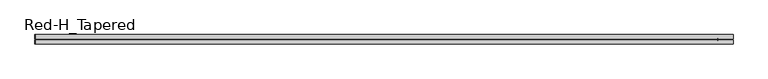
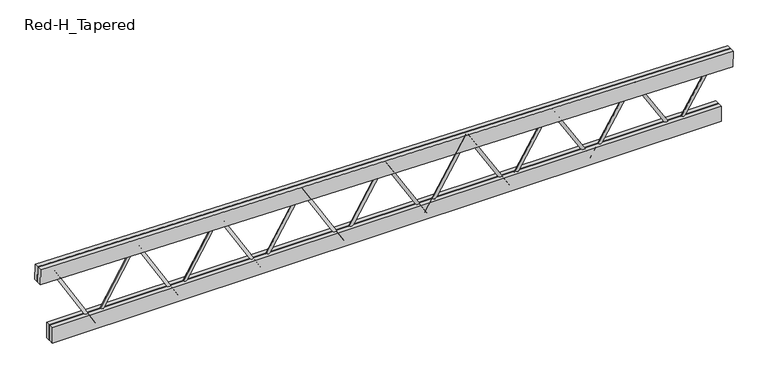
"""IFC4 building model written with IfcOpenShell, lengths in millimetres: beam geometry, Construction_Frames_RedBuilt_Openweb_Red-H_Tapered : Red-H_Tapered."""

from ifc_helpers import new_model, si_unit, point, frame, origin, origin_2d, place, context, project, spatial, polyline, circle_curve, trimmed, segment, composite_curve, outline, extrude, source, transform, mapped, element, save


def red_h_tapered_d62e6985(model_context):
    return source(origin(), model_context, "Body", "SweptSolid", [
        extrude(outline(composite_curve([segment(trimmed(circle_curve(origin_2d(), 12.7), [point((0.0, 12.7000001))], [point((0.0, -12.6999999))], False, "CARTESIAN"), True, "CONTINUOUS"), segment(trimmed(circle_curve(origin_2d(), 12.7), [point((0.0, -12.6999999))], [point((0.0, 12.7000001))], False, "CARTESIAN"), True, "CONTINUOUS")], self_intersect=False)), frame((2528.0870801, 0.0, -367.0101562), z_axis=(0.5258362965006711, 0.0, 0.8505857918413982), x_axis=(0.0, -1.0, 0.0)), (0.0, 0.0, 1.0), 686.8207835),
        extrude(outline(composite_curve([segment(trimmed(circle_curve(origin_2d(), 12.7), [point((0.0, -12.7))], [point((0.0, 12.7))], False, "CARTESIAN"), True, "CONTINUOUS"), segment(trimmed(circle_curve(origin_2d(), 12.7), [point((0.0, 12.7))], [point((0.0, -12.7))], False, "CARTESIAN"), True, "CONTINUOUS")], self_intersect=False)), frame((2528.0870801, 0.0, -367.0101562), z_axis=(-0.5232628307929019, 0.0, 0.8521713500878794), x_axis=(0.0, -1.0, 0.0)), (0.0, 0.0, 1.0), 690.1986457),
        extrude(outline(composite_curve([segment(trimmed(circle_curve(origin_2d(), 12.7), [point((0.0, 12.7000001))], [point((0.0, -12.6999999))], False, "CARTESIAN"), True, "CONTINUOUS"), segment(trimmed(circle_curve(origin_2d(), 12.7), [point((0.0, -12.6999999))], [point((0.0, 12.7000001))], False, "CARTESIAN"), True, "CONTINUOUS")], self_intersect=False)), frame((1805.7764858, 0.0, -367.0101562), z_axis=(0.5232628307929034, 0.0, 0.8521713500878785), x_axis=(0.0, -1.0, 0.0)), (0.0, 0.0, 1.0), 690.1986457),
        extrude(outline(composite_curve([segment(trimmed(circle_curve(origin_2d(), 12.7), [point((0.0, -12.7000001))], [point((0.0, 12.7))], False, "CARTESIAN"), True, "CONTINUOUS"), segment(trimmed(circle_curve(origin_2d(), 12.7), [point((0.0, 12.7))], [point((0.0, -12.7000001))], False, "CARTESIAN"), True, "CONTINUOUS")], self_intersect=False)), frame((1805.7764858, 0.0, -367.0101562), z_axis=(-0.5207097434413256, 0.0, 0.8537337776410565), x_axis=(0.0, -1.0, 0.0)), (0.0, 0.0, 1.0), 693.5827526),
        extrude(outline(composite_curve([segment(trimmed(circle_curve(origin_2d(), 12.7), [point((0.0, 12.7000001))], [point((0.0, -12.7))], False, "CARTESIAN"), True, "CONTINUOUS"), segment(trimmed(circle_curve(origin_2d(), 12.7), [point((0.0, -12.7))], [point((0.0, 12.7000001))], False, "CARTESIAN"), True, "CONTINUOUS")], self_intersect=False)), frame((1083.4658915, 0.0, -367.0101562), z_axis=(0.5207097434413247, 0.0, 0.8537337776410572), x_axis=(0.0, -1.0, 0.0)), (0.0, 0.0, 1.0), 693.5827526),
        extrude(outline(composite_curve([segment(trimmed(circle_curve(origin_2d(), 12.7), [point((0.0, -12.7))], [point((0.0, 12.6999999))], False, "CARTESIAN"), True, "CONTINUOUS"), segment(trimmed(circle_curve(origin_2d(), 12.7), [point((0.0, 12.6999999))], [point((0.0, -12.7))], False, "CARTESIAN"), True, "CONTINUOUS")], self_intersect=False)), frame((1083.4658915, 0.0, -367.0101562), z_axis=(-0.5181768738610981, 0.0, 0.8552734810547675), x_axis=(0.0, -1.0, 0.0)), (0.0, 0.0, 1.0), 696.9730132),
        extrude(outline(composite_curve([segment(trimmed(circle_curve(origin_2d(), 12.7), [point((0.0, 12.7))], [point((0.0, -12.6999999))], False, "CARTESIAN"), True, "CONTINUOUS"), segment(trimmed(circle_curve(origin_2d(), 12.7), [point((0.0, -12.6999999))], [point((0.0, 12.7))], False, "CARTESIAN"), True, "CONTINUOUS")], self_intersect=False)), frame((361.1552972, 0.0, -367.0101562), z_axis=(0.5181768738610981, 0.0, 0.8552734810547675), x_axis=(0.0, -1.0, 0.0)), (0.0, 0.0, 1.0), 696.9730132),
        extrude(outline(composite_curve([segment(trimmed(circle_curve(origin_2d(), 12.7), [point((0.0, -12.7))], [point((0.0, 12.7))], False, "CARTESIAN"), True, "CONTINUOUS"), segment(trimmed(circle_curve(origin_2d(), 12.7), [point((0.0, 12.7))], [point((0.0, -12.7))], False, "CARTESIAN"), True, "CONTINUOUS")], self_intersect=False)), frame((361.1552972, 0.0, -367.0101562), z_axis=(-0.5156640610107673, 0.0, 0.8567908590676512), x_axis=(0.0, -1.0, 0.0)), (0.0, 0.0, 1.0), 700.3693382),
        extrude(outline(composite_curve([segment(trimmed(circle_curve(origin_2d(), 12.7), [point((0.0, -12.7))], [point((0.0, 12.7))], False, "CARTESIAN"), True, "CONTINUOUS"), segment(trimmed(circle_curve(origin_2d(), 12.7), [point((0.0, 12.7))], [point((0.0, -12.7))], False, "CARTESIAN"), True, "CONTINUOUS")], self_intersect=False)), frame((-361.1552972, 0.0, -367.0101562), z_axis=(0.5156640610107361, 0.0, 0.8567908590676699), x_axis=(0.0, -1.0, 0.0)), (0.0, 0.0, 1.0), 700.3693382),
        extrude(outline(composite_curve([segment(trimmed(circle_curve(origin_2d(), 12.7), [point((0.0, 12.7))], [point((0.0, -12.7))], False, "CARTESIAN"), True, "CONTINUOUS"), segment(trimmed(circle_curve(origin_2d(), 12.7), [point((0.0, -12.7))], [point((0.0, 12.7))], False, "CARTESIAN"), True, "CONTINUOUS")], self_intersect=False)), frame((-361.1552972, 0.0, -367.0101562), z_axis=(-0.5131711434938878, 0.0, 0.8582863027482005), x_axis=(0.0, -1.0, 0.0)), (0.0, 0.0, 1.0), 703.7716398),
        extrude(outline(composite_curve([segment(trimmed(circle_curve(origin_2d(), 12.7), [point((0.0, -12.6999999))], [point((0.0, 12.7000001))], False, "CARTESIAN"), True, "CONTINUOUS"), segment(trimmed(circle_curve(origin_2d(), 12.7), [point((0.0, 12.7000001))], [point((0.0, -12.6999999))], False, "CARTESIAN"), True, "CONTINUOUS")], self_intersect=False)), frame((-1083.4658915, 0.0, -367.0101562), z_axis=(0.5131711434938859, 0.0, 0.8582863027482016), x_axis=(0.0, -1.0, 0.0)), (0.0, 0.0, 1.0), 703.7716398),
        extrude(outline(composite_curve([segment(trimmed(circle_curve(origin_2d(), 12.7), [point((0.0, 12.7))], [point((0.0, -12.7))], False, "CARTESIAN"), True, "CONTINUOUS"), segment(trimmed(circle_curve(origin_2d(), 12.7), [point((0.0, -12.7))], [point((0.0, 12.7))], False, "CARTESIAN"), True, "CONTINUOUS")], self_intersect=False)), frame((-1083.4658915, 0.0, -367.0101562), z_axis=(-0.5106979596558443, 0.0, 0.8597601956379219), x_axis=(0.0, -1.0, 0.0)), (0.0, 0.0, 1.0), 707.1798317),
        extrude(outline(composite_curve([segment(trimmed(circle_curve(origin_2d(), 12.7), [point((0.0, -12.7))], [point((0.0, 12.7))], False, "CARTESIAN"), True, "CONTINUOUS"), segment(trimmed(circle_curve(origin_2d(), 12.7), [point((0.0, 12.7))], [point((0.0, -12.7))], False, "CARTESIAN"), True, "CONTINUOUS")], self_intersect=False)), frame((-1805.7764858, 0.0, -367.0101562), z_axis=(0.5106979596558576, 0.0, 0.859760195637914), x_axis=(0.0, -1.0, 0.0)), (0.0, 0.0, 1.0), 707.1798317),
        extrude(outline(composite_curve([segment(trimmed(circle_curve(origin_2d(), 12.7), [point((0.0, 12.7))], [point((0.0, -12.7))], False, "CARTESIAN"), True, "CONTINUOUS"), segment(trimmed(circle_curve(origin_2d(), 12.7), [point((0.0, -12.7))], [point((0.0, 12.7))], False, "CARTESIAN"), True, "CONTINUOUS")], self_intersect=False)), frame((-1805.7764858, 0.0, -367.0101562), z_axis=(-0.5082443476755641, 0.0, 0.8612129138928656), x_axis=(0.0, -1.0, 0.0)), (0.0, 0.0, 1.0), 710.5938292),
        extrude(outline(composite_curve([segment(trimmed(circle_curve(origin_2d(), 12.7), [point((0.0, -12.7000001))], [point((0.0, 12.7))], False, "CARTESIAN"), True, "CONTINUOUS"), segment(trimmed(circle_curve(origin_2d(), 12.7), [point((0.0, 12.7))], [point((0.0, -12.7000001))], False, "CARTESIAN"), True, "CONTINUOUS")], self_intersect=False)), frame((-2528.0870801, 0.0, -367.0101562), z_axis=(0.5082443476755543, 0.0, 0.8612129138928715), x_axis=(0.0, -1.0, 0.0)), (0.0, 0.0, 1.0), 710.5938292),
        extrude(outline(composite_curve([segment(trimmed(circle_curve(origin_2d(), 12.7), [point((0.0, 12.6999999))], [point((0.0, -12.7))], False, "CARTESIAN"), True, "CONTINUOUS"), segment(trimmed(circle_curve(origin_2d(), 12.7), [point((0.0, -12.7))], [point((0.0, 12.6999999))], False, "CARTESIAN"), True, "CONTINUOUS")], self_intersect=False)), frame((-2528.0870801, 0.0, -367.0101562), z_axis=(-0.505810145652781, 0.0, 0.8626448264231997), x_axis=(0.0, -1.0, 0.0)), (0.0, 0.0, 1.0), 714.0135489),
        extrude(outline(polyline([(-2914.6423773, -41.275), (-2914.6423773, -3.175), (2914.6423773, -3.175), (2914.6423773, -41.275), (-2914.6423773, -41.275)])), frame((0.0, 0.0, -386.0601562), z_axis=(0.0, 0.0, 1.0), x_axis=(1.0, 0.0, 0.0)), (0.0, 0.0, 1.0), 139.7),
        extrude(outline(polyline([(-2914.6423773, 3.175), (-2914.6423773, 41.275), (2914.6423773, 41.275), (2914.6423773, 3.175), (-2914.6423773, 3.175)])), frame((0.0, 0.0, -386.0601562), z_axis=(0.0, 0.0, 1.0), x_axis=(1.0, 0.0, 0.0)), (0.0, 0.0, 1.0), 139.7),
        extrude(outline(polyline([(0.0, -38.1), (0.0, 0.0), (6033.340275, 0.0), (6033.340275, -38.1), (0.0, -38.1)])), frame((-3018.5948917, -3.175, 185.459653), z_axis=(0.016839759630315046, 0.0, 0.999858201194346), x_axis=(0.999858201194346, 0.0, -0.016839759630315046)), (0.0, 0.0, 1.0), 139.7),
        extrude(outline(polyline([(0.0, -38.1), (0.0, 0.0), (6033.340275, 0.0), (6033.340275, -38.1), (0.0, -38.1)])), frame((-3018.5948917, 41.275, 185.459653), z_axis=(0.016839759630315046, 0.0, 0.999858201194346), x_axis=(0.999858201194346, 0.0, -0.016839759630315046)), (0.0, 0.0, 1.0), 139.7),
    ])


if __name__ == "__main__":
    model = new_model("IFC4")
    model_context = context("Model", 3, world=origin())
    ifc_project = project(units=[si_unit("LENGTHUNIT", "METRE", prefix="MILLI")], contexts=[model_context])
    site = spatial("IfcSite", under=ifc_project)
    building = spatial("IfcBuilding", under=site)
    placement = place(None, origin())
    red_h_tapered_shape = red_h_tapered_d62e6985(model_context)
    element("IfcBeam", 1, ObjectType="Construction_Frames_RedBuilt_Openweb_Red-H_Tapered : Red-H_Tapered", at=placement, inside=building, context=model_context, shape_type="MappedRepresentation", body=[
        mapped(red_h_tapered_shape, transform((0.0, 0.0, 0.0), x_axis=(1.0, 0.0, 0.0), y_axis=(0.0, 1.0, 0.0), z_axis=(0.0, 0.0, 1.0))),
    ])
    save(model, "model.ifc")

# Revit data of these elements
# Type "Construction_Frames_RedBuilt_Openweb_Red-H_Tapered : Red-H_Tapered"
#   Youtube clip = ""
#   Weight Net (Kg) = "0"
#   Webs = "Up to 2\" diameter tubular steel"
#   Uniformat II Description = ""
#   Uniformat II Code = ""
#   Uniclass 2015 Name = "Softwood trusses"
#   Uniclass 2015 Code = "Pr_20_85_90_81"
#   Uniclass 2.0 Description = "Structural Framing Systems"
#   Uniclass 2.0 Code = "SS-15-10-75"
#   Uniclass 1.4 Description = "Trusses"
#   Uniclass 1.4 Code = "L3523"
#   UNSPSC Code = "30103606"
#   Technical description = "http://www.redbuilt.com/reference/literature-and-other-resources"
#   Region South America = "None"
#   Region Oceania = "None"
#   Region North America = "US"
#   Region Middle East = "None"
#   Region Europe = "None"
#   Region Asia = "None"
#   Region Antarctica = "None"
#   Region Africa = "None"
#   QR code = "http://bimobject.com/redbuilt/product/redbuilt-0003"
#   Product url = "http://www.redbuilt.com/products/default.aspx?id=2"
#   Product group = "Wood Trusses"
#   Product family = "Construction"
#   Product data url = "https://bimobject.com/redbuilt/product/redbuilt-0003"
#   Product certification = ""
#   Product SKU = "redbuilt-0003"
#   Product Page URL = "http://www.redbuilt.com/commercial-systems/red-m-red-h-open-web-trusses"
#   Product Guid = "2c5793f2-6ffb-4665-b825-cf90c048e711"
#   Product Documentation Link = "http://www.redbuilt.com/documents/OW_Guide_2017_07_LowRes_wLinks.pdf"
#   OmniClass Description = "Wood Trusses"
#   OmniClass Code = "23-13 35 19 13 17"
#   NBS Reference Description = ""
#   NBS Reference Code = ""
#   Material secondary = "Steel"
#   Material main = "CHARRED WOOD"
#   Masterformat 2014 Description = "Metal-Web Wood Joists"
#   Masterformat 2014 Code = "06 17 36"
#   Manufacturer name = "RedBuilt"
#   Manufacturer country = "United States"
#   Installation instructions = "http://www.redbuilt.com/documents/Installation_Sheets_Open-Web.pdf"
#   IFC Classification = ""
#   EAN code = ""
#   Design country = "United States"
#   Product Information = "http://redbuilt.com/products/default.aspx?id=2"
#   Model = "Red-H-Tapered"
#   Manufacturer URL = "http://redbuilt.com/"
#   Manufacturer = "RedBuilt™"
#   Description = "Open Web Truss"
#   Date of publishing = "8/17/2010"
#   Contact us = "http://redbuilt.com/contact/"
#   Chords = "Double 1½\" x 5½\" MSR lumber"
#   COBIe Type Category = ""
#   Brand url = "http://www.redbuilt.com"
#   BIMobject main category code = "construction"
#   BIMobject main category = "Construction"
#   BIMobject category code = "construction-frames-trusses"
#   BIMobject category = "Frames & Trusses"
#   Web Radius = 0' - 0 1/2"
#   Web Layout Offset Start [instance default] = 0' - 5"
#   Web Layout Offset End [instance default] = 0' - 5"
#   Web Diameter = 0' - 1"
#   TotalLength [instance default] = 20' - 0"
#   Span Minimum = 4' - 0"
#   Span Maximum = 70' - 0"
#   Span Limit [instance default] = 20' - 0"
#   Nominal width = 0' - 0"
#   Nominal height = 0' - 0"
#   Inner Depth Top [instance default] = 0' - 2.76372"
#   Depth Start [instance default] = 6' - 0"
#   Top Chord Length [instance default] = 20' - 1.19701"
#   TC Extension Start Aux [instance default] = 0' - 0"
#   TC Extension End Aux [instance default] = 0' - 0"
#   T-B Chord Length Difference L [instance default] = 0' - 4"
#   T-B Chord Length Difference [instance default] = 0' - 4"
#   Height 2 [instance default] = 6' - 0"
#   Depth Minimum at Wall = 2' - 0"
#   Depth Maximum at Wall = 6' - 0"
#   Depth Lower End [instance default] = 2' - 0"
#   Depth Higher End [instance default] = 6' - 0"
#   Depth End [instance default] = 2' - 0"
#   Depth 2 [instance default] = 2' - 0"
#   Chord Width = 0' - 3 1/4"
#   Chord Thickness = 0' - 1 1/2"
#   Chord Depth = 0' - 5 1/2"
#   Offset Start [instance default] = 0' - 0"
#   TC Extension Start [instance default] = 0' - 0"
#   End Panel = 0' - 5"
#   Offset End [instance default] = 0' - 0"
#   TC Extension End [instance default] = 0' - 0"
#   Length [instance default] = 20' - 0"
#   Angle [instance default] = 5.71059°
#   Span Limit Warning [instance default] = no
#   Edition number = 1
#   Top Bearing Start [instance default] = yes
#   Top Bearing End [instance default] = yes
#   Bottom Bearing Start [instance default] = no
#   Bottom Bearing End [instance default] = no
#   8 Panels [instance default] = yes
#   16 Panels [instance default] = no
#   12 Panels [instance default] = no
#   Web Material = RedBuilt-Steel, Galvanized
#   Clip Material = RedBuilt-Steel, Galvanized
#   Chords Material = WOOD-OAKFIRE
#   URL = ""
#   Assembly Code = ""
# Element 1 (IfcBeam, "Construction_Frames_RedBuilt_Openweb_Red-H_Tapered : Red-H_Tapered")
#   TotalLength = 19' - 9.4994"
#   Span Limit = 19' - 9.4994"
#   Inner Depth Top = 0' - 2.75039"
#   Depth Start = 5' - 0"
#   Top Chord Length = 19' - 9.53308"
#   Height 2 = 5' - 0"
#   Depth Higher End = 5' - 0"
#   Depth 2 = 0' - 4"
#   Angle = 0.964893°
#   Materials on its faces: "RedBuilt-Steel, Galvanized", "WOOD-OAKFIRE"
# Materials
#   "RedBuilt-Steel, Galvanized": class "Metal", colour RGB 164 172 176, transparency 0, Manufacturer = "RedBuilt. LLC", Comments = "Openweb Metal Web", URL = "http://www.redbuilt.com/", Description = "Galvanized steel", Cost = 0
#   "WOOD-OAKFIRE": class "Wood", colour RGB 198 202 183, transparency 0, Description = "Generic wood", Cost = 0
